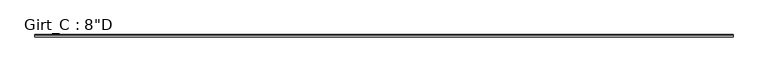
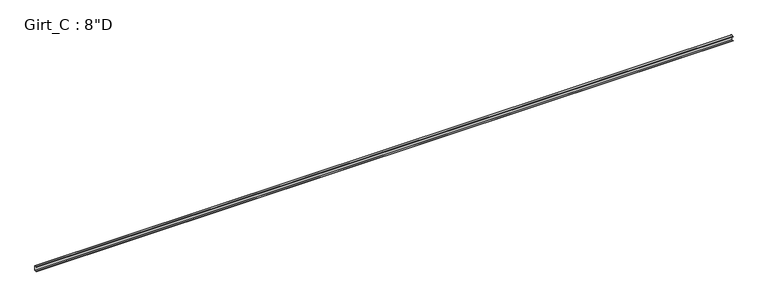
"""IFC4 building model written with IfcOpenShell, lengths in millimetres: beam geometry."""

import ifcopenshell
import ifcopenshell.guid

model = None  # the IFC model being written
_history = None  # IfcOwnerHistory: only IFC2X3 demands one
_inside = {}  # id of a spatial element -> (the spatial element, [elements in it])
_under = {}  # id of a project, library or spatial element -> (it, [spatial elements below it])
_declared = {}  # id of a project -> (the project, [libraries it declares])
_typed = {}  # id of a type object -> (the type object, [elements of that type])
_made_of = {}  # id of a material, layer set ... -> (it, [elements and type objects made of it])


def new_model(schema):
    """Start an empty IFC model of exactly this schema.

    Asked for "IFC4X3", IfcOpenShell would pick the latest addendum, in which some entities
    have other attributes; the version numbers below select the first issue.
    IFC2X3 requires an IfcOwnerHistory on every rooted entity: one is made here for all.
    """
    global model, _history
    if schema == "IFC4X3":
        model = ifcopenshell.file(schema_version=(4, 3, 0, 0))
    else:
        model = ifcopenshell.file(schema=schema)
    _inside.clear()
    _under.clear()
    _declared.clear()
    _typed.clear()
    _made_of.clear()
    _history = None
    if model.schema == "IFC2X3":
        org = make("IfcOrganization", Name="unknown")
        user = make(
            "IfcPersonAndOrganization",
            ThePerson=make("IfcPerson", FamilyName="unknown"),
            TheOrganization=org,
        )
        app = make(
            "IfcApplication",
            ApplicationDeveloper=org,
            Version="unknown",
            ApplicationFullName="unknown",
            ApplicationIdentifier="unknown",
        )
        _history = make(
            "IfcOwnerHistory",
            OwningUser=user,
            OwningApplication=app,
            ChangeAction="ADDED",
            CreationDate=0,
        )
    return model


def make(cls, **values):
    """One entity of the class cls with the attributes given. An attribute that is None is left unset."""
    return model.create_entity(
        cls, **{name: value for name, value in values.items() if value is not None}
    )


def rooted(cls, **values):
    """An entity with a GlobalId (a new one), such as an element, a storey or a relation."""
    return make(cls, GlobalId=ifcopenshell.guid.new(), OwnerHistory=_history, **values)


def si_unit(unit_type, name, prefix=None):
    """IfcSIUnit, for example si_unit("LENGTHUNIT", "METRE", prefix="MILLI")."""
    return make("IfcSIUnit", UnitType=unit_type, Prefix=prefix, Name=name)


def assignment(units):
    """IfcUnitAssignment: the units of a project."""
    return None if units is None else make("IfcUnitAssignment", Units=units)


def point(xyz):
    """IfcCartesianPoint."""
    return None if xyz is None else make("IfcCartesianPoint", Coordinates=xyz)


def direction(xyz):
    """IfcDirection."""
    return None if xyz is None else make("IfcDirection", DirectionRatios=xyz)


def frame(location, z_axis=None, x_axis=None):
    """IfcAxis2Placement3D, a coordinate frame: its origin and axes. An axis left out is left unset."""
    return make(
        "IfcAxis2Placement3D",
        Location=point(location),
        Axis=direction(z_axis),
        RefDirection=direction(x_axis),
    )


def frame_2d(location, x_axis=None):
    """IfcAxis2Placement2D, a coordinate frame in the plane: its origin and x axis."""
    return make(
        "IfcAxis2Placement2D", Location=point(location), RefDirection=direction(x_axis)
    )


def origin():
    """The frame at (0, 0, 0) with its axes left unset."""
    return frame((0.0, 0.0, 0.0))


def place(relative_to, where):
    """IfcLocalPlacement: puts the frame where relative to a parent placement (None: the world)."""
    return make(
        "IfcLocalPlacement", PlacementRelTo=relative_to, RelativePlacement=where
    )


def context(
    kind, dimensions, precision=None, world=None, true_north=None, identifier=None
):
    """IfcGeometricRepresentationContext, for example the 3D "Model" context."""
    return make(
        "IfcGeometricRepresentationContext",
        ContextIdentifier=identifier,
        ContextType=kind,
        CoordinateSpaceDimension=dimensions,
        Precision=precision,
        WorldCoordinateSystem=world,
        TrueNorth=true_north,
    )


def project(units=None, contexts=None):
    """IfcProject with its units and contexts."""
    return rooted(
        "IfcProject",
        Name="project",
        RepresentationContexts=contexts,
        UnitsInContext=assignment(units),
    )


def spatial(cls, under=None, at=None, **own):
    """A site, building, storey or space (cls), placed at a placement, below another one or the project."""
    s = rooted(cls, ObjectPlacement=at, **own)
    if under is not None:
        _under.setdefault(under.id(), (under, []))[1].append(s)
    return s


def polyline(points):
    """IfcPolyline through the points."""
    return make("IfcPolyline", Points=[point(p) for p in points])


def circle_curve(where, radius):
    """IfcCircle in the frame where."""
    return make("IfcCircle", Position=where, Radius=radius)


def trimmed(basis, trim1, trim2, sense, master):
    """IfcTrimmedCurve: the piece of a basis curve between two trims."""
    return make(
        "IfcTrimmedCurve",
        BasisCurve=basis,
        Trim1=trim1,
        Trim2=trim2,
        SenseAgreement=sense,
        MasterRepresentation=master,
    )


def segment(curve, same_sense, transition):
    """IfcCompositeCurveSegment."""
    return make(
        "IfcCompositeCurveSegment",
        Transition=transition,
        SameSense=same_sense,
        ParentCurve=curve,
    )


def composite_curve(segments, self_intersect=None):
    """IfcCompositeCurve: segments joined end to end."""
    return make("IfcCompositeCurve", Segments=segments, SelfIntersect=self_intersect)


def outline(outer, holes=None, kind="AREA"):
    """IfcArbitraryClosedProfileDef: a profile drawn as a closed curve; with holes, ...WithVoids."""
    if holes is None:
        return make("IfcArbitraryClosedProfileDef", ProfileType=kind, OuterCurve=outer)
    return make(
        "IfcArbitraryProfileDefWithVoids",
        ProfileType=kind,
        OuterCurve=outer,
        InnerCurves=holes,
    )


def extrude(swept, where, along, depth):
    """IfcExtrudedAreaSolid: the profile swept, set in the frame where, extruded along a direction by depth."""
    return make(
        "IfcExtrudedAreaSolid",
        SweptArea=swept,
        Position=where,
        ExtrudedDirection=direction(along),
        Depth=depth,
    )


def shape(context_of_items, identifier, shape_type, items):
    """IfcShapeRepresentation: the items that make up one representation, for example the "Body"."""
    return make(
        "IfcShapeRepresentation",
        ContextOfItems=context_of_items,
        RepresentationIdentifier=identifier,
        RepresentationType=shape_type,
        Items=items,
    )


def source(mapping_origin, context_of_items, identifier, shape_type, items):
    """IfcRepresentationMap: a shape defined once, which mapped items show again and again."""
    return make(
        "IfcRepresentationMap",
        MappingOrigin=mapping_origin,
        MappedRepresentation=shape(context_of_items, identifier, shape_type, items),
    )


def transform(
    local_origin,
    x_axis=None,
    y_axis=None,
    z_axis=None,
    scale=None,
    scale2=None,
    scale3=None,
    uniform=True,
):
    """IfcCartesianTransformationOperator3D, or its non-uniform kind. x_axis, y_axis, z_axis: its Axis1, 2, 3."""
    if uniform:
        return make(
            "IfcCartesianTransformationOperator3D",
            Axis1=direction(x_axis),
            Axis2=direction(y_axis),
            LocalOrigin=point(local_origin),
            Scale=scale,
            Axis3=direction(z_axis),
        )
    return make(
        "IfcCartesianTransformationOperator3DnonUniform",
        Axis1=direction(x_axis),
        Axis2=direction(y_axis),
        LocalOrigin=point(local_origin),
        Scale=scale,
        Axis3=direction(z_axis),
        Scale2=scale2,
        Scale3=scale3,
    )


def mapped(mapping_source, mapping_target):
    """IfcMappedItem: shows the shape of a source again, moved by a transform."""
    return make(
        "IfcMappedItem", MappingSource=mapping_source, MappingTarget=mapping_target
    )


def made_of(thing, what):
    """Note that an element or type object is made of a material, layer set ...; save() writes the relation."""
    if what is not None:
        _made_of.setdefault(what.id(), (what, []))[1].append(thing)
    return thing


def element(
    cls,
    number,
    at=None,
    inside=None,
    cuts=None,
    type_object=None,
    material=None,
    context=None,
    identifier="Body",
    shape_type=None,
    held_by="IfcProductDefinitionShape",
    body=None,
    shapes=None,
    **own,
):
    """One element of the class cls, such as IfcWall. Its Tag is "e" and its number.

    at: its placement. inside: the storey or other place that contains it. cuts: it is an
    opening in that element (IfcRelVoidsElement). A single representation is given by context,
    identifier, shape_type and body (its items); several are given by shapes. held_by: the class
    of the entity that holds the representations. save() writes the other relations.
    """
    e = rooted(cls, Tag="e%d" % number, ObjectPlacement=at, **own)
    if body is not None:
        shapes = [shape(context, identifier, shape_type, body)]
    if shapes is not None:
        e.Representation = make(held_by, Representations=shapes)
    if inside is not None:
        _inside.setdefault(inside.id(), (inside, []))[1].append(e)
    if cuts is not None:
        rooted(
            "IfcRelVoidsElement", RelatingBuildingElement=cuts, RelatedOpeningElement=e
        )
    if type_object is not None:
        _typed.setdefault(type_object.id(), (type_object, []))[1].append(e)
    return made_of(e, material)


def aggregate(whole, parts):
    """IfcRelAggregates: a whole, such as a stair, and the parts it consists of."""
    return rooted("IfcRelAggregates", RelatingObject=whole, RelatedObjects=parts)


def save(model, path):
    """Write the relations noted so far, then the file.

    IfcRelAggregates (storeys below a building ...), IfcRelContainedInSpatialStructure (elements
    in a storey), IfcRelDefinesByType, IfcRelAssociatesMaterial and IfcRelDeclares: one each for
    every whole, place, type object, material and project.
    """
    for whole, parts in _under.values():
        aggregate(whole, parts)
    for where, things in _inside.values():
        rooted(
            "IfcRelContainedInSpatialStructure",
            RelatedElements=things,
            RelatingStructure=where,
        )
    for kind, things in _typed.values():
        rooted("IfcRelDefinesByType", RelatedObjects=things, RelatingType=kind)
    for what, things in _made_of.values():
        rooted("IfcRelAssociatesMaterial", RelatedObjects=things, RelatingMaterial=what)
    for by, libraries in _declared.values():
        rooted("IfcRelDeclares", RelatingContext=by, RelatedDefinitions=libraries)
    model.write(path)


def beam_88a5fd93(model_context):
    return source(origin(), model_context, "Body", "SweptSolid", [
        extrude(outline(composite_curve([segment(polyline([(-87.5109375, 101.6), (-3.3734375, 101.6)]), True, "CONTINUOUS"), segment(trimmed(circle_curve(frame_2d((-3.3734375, 96.8375)), 4.7625), [point((-3.3734375, 101.6))], [point((1.3890625, 96.8375))], False, "CARTESIAN"), True, "CONTINUOUS"), segment(polyline([(1.3890625, 96.8375), (1.3890625, -96.8375)]), True, "CONTINUOUS"), segment(trimmed(circle_curve(frame_2d((-3.3734375, -96.8375)), 4.7625), [point((1.3890625, -96.8375))], [point((-3.3734375, -101.6))], False, "CARTESIAN"), True, "CONTINUOUS"), segment(polyline([(-3.3734375, -101.6), (-87.5109375, -101.6), (-99.7792647, -86.979177), (-97.6510975, -85.1934327), (-86.2154765, -98.821875), (-3.2694106, -98.821875)]), True, "CONTINUOUS"), segment(trimmed(circle_curve(frame_2d((-3.3748024, -96.8389339)), 1.9857399), [point((-3.2694106, -98.821875))], [point((-1.3890625, -96.8389339))], True, "CARTESIAN"), True, "CONTINUOUS"), segment(polyline([(-1.3890625, -96.8389339), (-1.3890625, 96.8381931)]), True, "CONTINUOUS"), segment(trimmed(circle_curve(frame_2d((-3.3741066, 96.8381931)), 1.9850441), [point((-1.3890625, 96.8381931))], [point((-3.3005807, 98.821875))], True, "CARTESIAN"), True, "CONTINUOUS"), segment(polyline([(-3.3005807, 98.821875), (-86.2154765, 98.821875), (-97.6278742, 85.221109), (-99.7560415, 87.0068534), (-87.5109375, 101.6)]), True, "CONTINUOUS")], self_intersect=False)), frame((-14148.6100916, 0.0, 0.0), z_axis=(1.0, 0.0, 0.0), x_axis=(0.0, 1.0, 0.0)), (0.0, 0.0, 1.0), 28297.2201833),
    ])


if __name__ == "__main__":
    model = new_model("IFC4")
    model_context = context("Model", 3, world=origin())
    ifc_project = project(units=[si_unit("LENGTHUNIT", "METRE", prefix="MILLI")], contexts=[model_context])
    site = spatial("IfcSite", under=ifc_project)
    building = spatial("IfcBuilding", under=site)
    placement = place(None, origin())
    beam_shape = beam_88a5fd93(model_context)
    element("IfcBeam", 1, ObjectType="Girt_C : 8\"D", at=placement, inside=building, context=model_context, shape_type="MappedRepresentation", body=[
        mapped(beam_shape, transform((0.0, 0.0, 0.0), x_axis=(1.0, 0.0, 0.0), y_axis=(0.0, 1.0, 0.0), z_axis=(0.0, 0.0, 1.0))),
    ])
    save(model, "model.ifc")

# Revit data of these elements
# Type "Girt_C : 8\"D"
#   half leg = 0' - 1 3/4"
#   Web_Thickness = 0' - 0 7/64"
#   Length [instance default] = 10' - 0"
#   Leg_1 = 0' - 3 1/2"
#   Height = 0' - 8"
#   Structural Material [instance default] = none
# Element 1 (IfcBeam, "Girt_C : 8\"D")
#   Structural Material = CEE' SECTION (8.0x3.5C - SEE STRUCT. DWGS)
#   Materials on its faces: "CEE' SECTION (8.0x3.5C - SEE STRUCT. DWGS)"
# Materials
#   "CEE' SECTION (8.0x3.5C - SEE STRUCT. DWGS)": class "Metal", colour RGB 137 146 153, transparency 0, Description = "Steel, mill finish", Cost = 0
